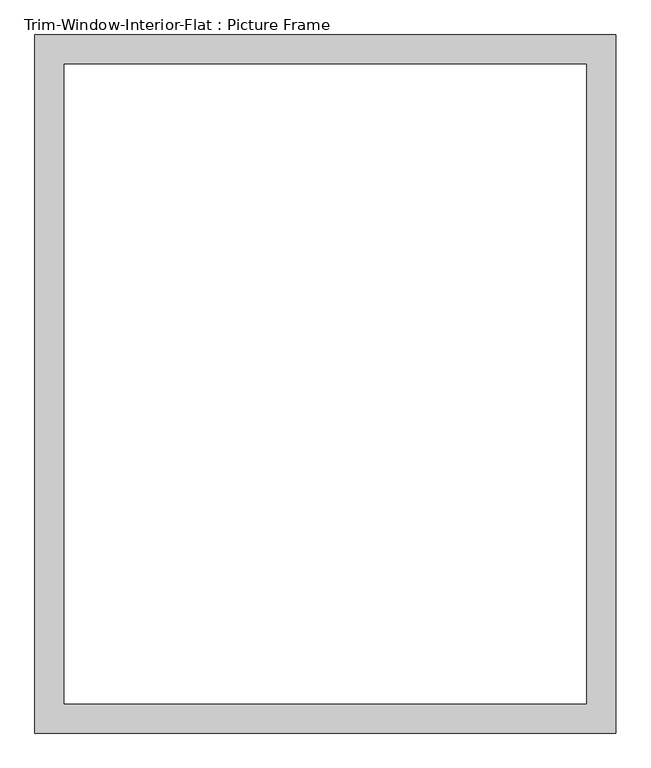
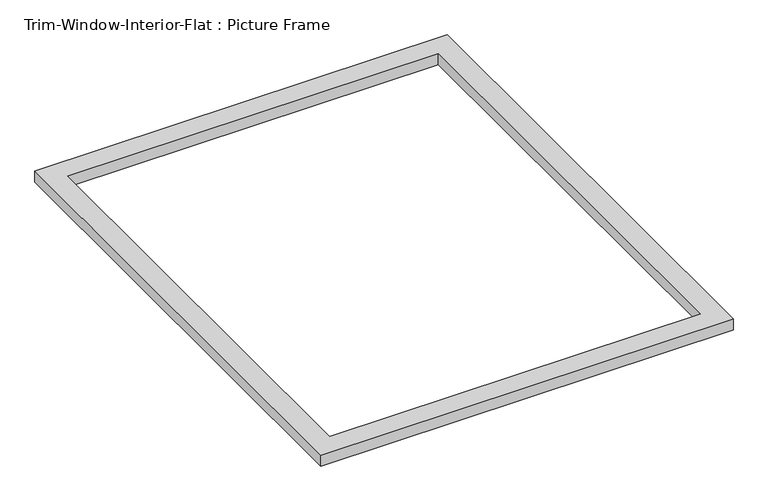
"""IFC4 building model written with IfcOpenShell, lengths in millimetres: proxy geometry, Trim-Window-Interior-Flat : Picture Frame."""

import ifcopenshell
import ifcopenshell.guid

model = None  # the IFC model being written
_history = None  # IfcOwnerHistory: only IFC2X3 demands one
_inside = {}  # id of a spatial element -> (the spatial element, [elements in it])
_under = {}  # id of a project, library or spatial element -> (it, [spatial elements below it])
_declared = {}  # id of a project -> (the project, [libraries it declares])
_typed = {}  # id of a type object -> (the type object, [elements of that type])
_made_of = {}  # id of a material, layer set ... -> (it, [elements and type objects made of it])


def new_model(schema):
    """Start an empty IFC model of exactly this schema.

    Asked for "IFC4X3", IfcOpenShell would pick the latest addendum, in which some entities
    have other attributes; the version numbers below select the first issue.
    IFC2X3 requires an IfcOwnerHistory on every rooted entity: one is made here for all.
    """
    global model, _history
    if schema == "IFC4X3":
        model = ifcopenshell.file(schema_version=(4, 3, 0, 0))
    else:
        model = ifcopenshell.file(schema=schema)
    _inside.clear()
    _under.clear()
    _declared.clear()
    _typed.clear()
    _made_of.clear()
    _history = None
    if model.schema == "IFC2X3":
        org = make("IfcOrganization", Name="unknown")
        user = make(
            "IfcPersonAndOrganization",
            ThePerson=make("IfcPerson", FamilyName="unknown"),
            TheOrganization=org,
        )
        app = make(
            "IfcApplication",
            ApplicationDeveloper=org,
            Version="unknown",
            ApplicationFullName="unknown",
            ApplicationIdentifier="unknown",
        )
        _history = make(
            "IfcOwnerHistory",
            OwningUser=user,
            OwningApplication=app,
            ChangeAction="ADDED",
            CreationDate=0,
        )
    return model


def make(cls, **values):
    """One entity of the class cls with the attributes given. An attribute that is None is left unset."""
    return model.create_entity(
        cls, **{name: value for name, value in values.items() if value is not None}
    )


def rooted(cls, **values):
    """An entity with a GlobalId (a new one), such as an element, a storey or a relation."""
    return make(cls, GlobalId=ifcopenshell.guid.new(), OwnerHistory=_history, **values)


def si_unit(unit_type, name, prefix=None):
    """IfcSIUnit, for example si_unit("LENGTHUNIT", "METRE", prefix="MILLI")."""
    return make("IfcSIUnit", UnitType=unit_type, Prefix=prefix, Name=name)


def assignment(units):
    """IfcUnitAssignment: the units of a project."""
    return None if units is None else make("IfcUnitAssignment", Units=units)


def point(xyz):
    """IfcCartesianPoint."""
    return None if xyz is None else make("IfcCartesianPoint", Coordinates=xyz)


def direction(xyz):
    """IfcDirection."""
    return None if xyz is None else make("IfcDirection", DirectionRatios=xyz)


def frame(location, z_axis=None, x_axis=None):
    """IfcAxis2Placement3D, a coordinate frame: its origin and axes. An axis left out is left unset."""
    return make(
        "IfcAxis2Placement3D",
        Location=point(location),
        Axis=direction(z_axis),
        RefDirection=direction(x_axis),
    )


def origin():
    """The frame at (0, 0, 0) with its axes left unset."""
    return frame((0.0, 0.0, 0.0))


def origin_with_axes():
    """The frame at (0, 0, 0) with the z axis (0, 0, 1) and the x axis (1, 0, 0) written out."""
    return frame((0.0, 0.0, 0.0), z_axis=(0.0, 0.0, 1.0), x_axis=(1.0, 0.0, 0.0))


def place(relative_to, where):
    """IfcLocalPlacement: puts the frame where relative to a parent placement (None: the world)."""
    return make(
        "IfcLocalPlacement", PlacementRelTo=relative_to, RelativePlacement=where
    )


def context(
    kind, dimensions, precision=None, world=None, true_north=None, identifier=None
):
    """IfcGeometricRepresentationContext, for example the 3D "Model" context."""
    return make(
        "IfcGeometricRepresentationContext",
        ContextIdentifier=identifier,
        ContextType=kind,
        CoordinateSpaceDimension=dimensions,
        Precision=precision,
        WorldCoordinateSystem=world,
        TrueNorth=true_north,
    )


def project(units=None, contexts=None):
    """IfcProject with its units and contexts."""
    return rooted(
        "IfcProject",
        Name="project",
        RepresentationContexts=contexts,
        UnitsInContext=assignment(units),
    )


def spatial(cls, under=None, at=None, **own):
    """A site, building, storey or space (cls), placed at a placement, below another one or the project."""
    s = rooted(cls, ObjectPlacement=at, **own)
    if under is not None:
        _under.setdefault(under.id(), (under, []))[1].append(s)
    return s


def polyline(points):
    """IfcPolyline through the points."""
    return make("IfcPolyline", Points=[point(p) for p in points])


def outline(outer, holes=None, kind="AREA"):
    """IfcArbitraryClosedProfileDef: a profile drawn as a closed curve; with holes, ...WithVoids."""
    if holes is None:
        return make("IfcArbitraryClosedProfileDef", ProfileType=kind, OuterCurve=outer)
    return make(
        "IfcArbitraryProfileDefWithVoids",
        ProfileType=kind,
        OuterCurve=outer,
        InnerCurves=holes,
    )


def extrude(swept, where, along, depth):
    """IfcExtrudedAreaSolid: the profile swept, set in the frame where, extruded along a direction by depth."""
    return make(
        "IfcExtrudedAreaSolid",
        SweptArea=swept,
        Position=where,
        ExtrudedDirection=direction(along),
        Depth=depth,
    )


def shape(context_of_items, identifier, shape_type, items):
    """IfcShapeRepresentation: the items that make up one representation, for example the "Body"."""
    return make(
        "IfcShapeRepresentation",
        ContextOfItems=context_of_items,
        RepresentationIdentifier=identifier,
        RepresentationType=shape_type,
        Items=items,
    )


def source(mapping_origin, context_of_items, identifier, shape_type, items):
    """IfcRepresentationMap: a shape defined once, which mapped items show again and again."""
    return make(
        "IfcRepresentationMap",
        MappingOrigin=mapping_origin,
        MappedRepresentation=shape(context_of_items, identifier, shape_type, items),
    )


def transform(
    local_origin,
    x_axis=None,
    y_axis=None,
    z_axis=None,
    scale=None,
    scale2=None,
    scale3=None,
    uniform=True,
):
    """IfcCartesianTransformationOperator3D, or its non-uniform kind. x_axis, y_axis, z_axis: its Axis1, 2, 3."""
    if uniform:
        return make(
            "IfcCartesianTransformationOperator3D",
            Axis1=direction(x_axis),
            Axis2=direction(y_axis),
            LocalOrigin=point(local_origin),
            Scale=scale,
            Axis3=direction(z_axis),
        )
    return make(
        "IfcCartesianTransformationOperator3DnonUniform",
        Axis1=direction(x_axis),
        Axis2=direction(y_axis),
        LocalOrigin=point(local_origin),
        Scale=scale,
        Axis3=direction(z_axis),
        Scale2=scale2,
        Scale3=scale3,
    )


def mapped(mapping_source, mapping_target):
    """IfcMappedItem: shows the shape of a source again, moved by a transform."""
    return make(
        "IfcMappedItem", MappingSource=mapping_source, MappingTarget=mapping_target
    )


def made_of(thing, what):
    """Note that an element or type object is made of a material, layer set ...; save() writes the relation."""
    if what is not None:
        _made_of.setdefault(what.id(), (what, []))[1].append(thing)
    return thing


def element(
    cls,
    number,
    at=None,
    inside=None,
    cuts=None,
    type_object=None,
    material=None,
    context=None,
    identifier="Body",
    shape_type=None,
    held_by="IfcProductDefinitionShape",
    body=None,
    shapes=None,
    **own,
):
    """One element of the class cls, such as IfcWall. Its Tag is "e" and its number.

    at: its placement. inside: the storey or other place that contains it. cuts: it is an
    opening in that element (IfcRelVoidsElement). A single representation is given by context,
    identifier, shape_type and body (its items); several are given by shapes. held_by: the class
    of the entity that holds the representations. save() writes the other relations.
    """
    e = rooted(cls, Tag="e%d" % number, ObjectPlacement=at, **own)
    if body is not None:
        shapes = [shape(context, identifier, shape_type, body)]
    if shapes is not None:
        e.Representation = make(held_by, Representations=shapes)
    if inside is not None:
        _inside.setdefault(inside.id(), (inside, []))[1].append(e)
    if cuts is not None:
        rooted(
            "IfcRelVoidsElement", RelatingBuildingElement=cuts, RelatedOpeningElement=e
        )
    if type_object is not None:
        _typed.setdefault(type_object.id(), (type_object, []))[1].append(e)
    return made_of(e, material)


def aggregate(whole, parts):
    """IfcRelAggregates: a whole, such as a stair, and the parts it consists of."""
    return rooted("IfcRelAggregates", RelatingObject=whole, RelatedObjects=parts)


def save(model, path):
    """Write the relations noted so far, then the file.

    IfcRelAggregates (storeys below a building ...), IfcRelContainedInSpatialStructure (elements
    in a storey), IfcRelDefinesByType, IfcRelAssociatesMaterial and IfcRelDeclares: one each for
    every whole, place, type object, material and project.
    """
    for whole, parts in _under.values():
        aggregate(whole, parts)
    for where, things in _inside.values():
        rooted(
            "IfcRelContainedInSpatialStructure",
            RelatedElements=things,
            RelatingStructure=where,
        )
    for kind, things in _typed.values():
        rooted("IfcRelDefinesByType", RelatedObjects=things, RelatingType=kind)
    for what, things in _made_of.values():
        rooted("IfcRelAssociatesMaterial", RelatedObjects=things, RelatingMaterial=what)
    for by, libraries in _declared.values():
        rooted("IfcRelDeclares", RelatingContext=by, RelatedDefinitions=libraries)
    model.write(path)


def trim_window_interior_flat_picture_frame_bc4681b1(model_context):
    return source(origin(), model_context, "Body", "SweptSolid", [
        extrude(outline(polyline([(565.15, 44.45), (565.15, -1314.45), (-565.15, -1314.45), (-565.15, 44.45), (565.15, 44.45)]), holes=[polyline([(508.0, -12.7), (-508.0, -12.7), (-508.0, -1257.3), (508.0, -1257.3), (508.0, -12.7)])]), origin_with_axes(), (0.0, 0.0, 1.0), 31.75),
    ])


if __name__ == "__main__":
    model = new_model("IFC4")
    model_context = context("Model", 3, world=origin())
    ifc_project = project(units=[si_unit("LENGTHUNIT", "METRE", prefix="MILLI")], contexts=[model_context])
    site = spatial("IfcSite", under=ifc_project)
    building = spatial("IfcBuilding", under=site)
    placement = place(None, origin())
    trim_window_interior_flat_picture_frame_shape = trim_window_interior_flat_picture_frame_bc4681b1(model_context)
    element("IfcBuildingElementProxy", 1, Name="Trim-Window-Interior-Flat : Picture Frame", ObjectType="Trim-Window-Interior-Flat : Picture Frame", at=placement, inside=building, context=model_context, shape_type="MappedRepresentation", body=[
        mapped(trim_window_interior_flat_picture_frame_shape, transform((0.0, 0.0, 0.0), x_axis=(1.0, 0.0, 0.0), y_axis=(0.0, 1.0, 0.0), z_axis=(0.0, 0.0, 1.0))),
    ])
    save(model, "model.ifc")

# Revit data of these elements
# Type "Trim-Window-Interior-Flat : Picture Frame"
#   Trim Thickness_Picture Frame = 0' - 1 1/4"
#   Trim Width = 0' - 2 1/4"
#   Trim Thickness_with Sill = 0' - 0 3/4"
#   Sill Thickness = 0' - 1 1/4"
#   Opening Width [instance default] = 2' - 0"
#   Opening Height [instance default] = 3' - 0"
#   Default Elevation = 4' - 0"
#   Sill = no
#   Picture Frame = yes
#   Trim Material [instance default] = none
# Element 1 (IfcBuildingElementProxy, "Trim-Window-Interior-Flat : Picture Frame")
#   Opening Width = 3' - 5"
#   Opening Height = 4' - 2"
#   Trim Material = Wood - Stained
#   Materials on its faces: "Wood - Stained"
# Materials
#   "Wood - Stained": class "Wood", colour RGB 224 178 126, transparency 0, Cost = 0
